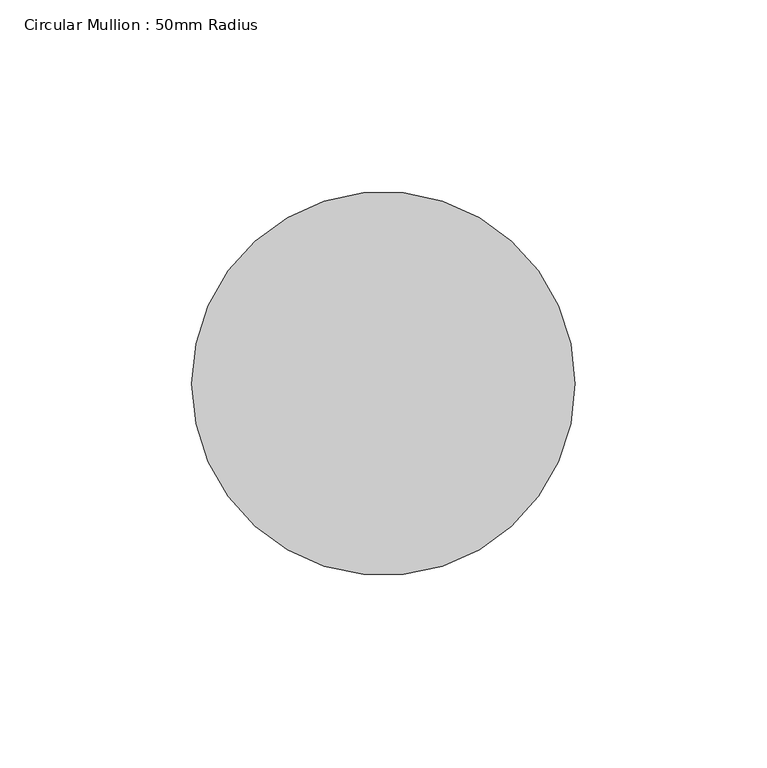
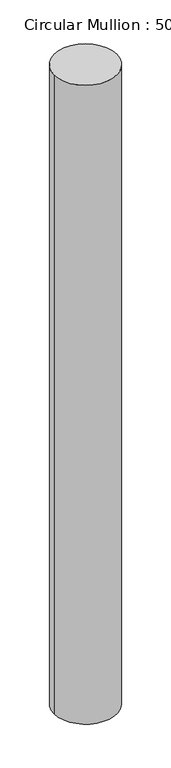
"""IFC4 building model written with IfcOpenShell, lengths in millimetres: member geometry, Circular Mullion : 50mm Radius."""

from ifc_helpers import new_model, si_unit, point, frame, origin, origin_2d, place, context, project, spatial, circle_curve, trimmed, segment, composite_curve, outline, extrude, source, transform, mapped, element, save


def circular_mullion_50mm_radius_108bae4b(model_context):
    return source(origin(), model_context, "Body", "SweptSolid", [
        extrude(outline(composite_curve([segment(trimmed(circle_curve(origin_2d(), 50.0), [point((50.0, 0.0))], [point((-50.0, 0.0))], False, "CARTESIAN"), True, "CONTINUOUS"), segment(trimmed(circle_curve(origin_2d(), 50.0), [point((-50.0, 0.0))], [point((50.0, 0.0))], False, "CARTESIAN"), True, "CONTINUOUS")], self_intersect=False)), frame((0.0, 0.0, -1076.8079908), z_axis=(0.0, 0.0, 1.0), x_axis=(1.0, 0.0, 0.0)), (0.0, 0.0, 1.0), 1076.8079908),
    ])


if __name__ == "__main__":
    model = new_model("IFC4")
    model_context = context("Model", 3, world=origin())
    ifc_project = project(units=[si_unit("LENGTHUNIT", "METRE", prefix="MILLI")], contexts=[model_context])
    site = spatial("IfcSite", under=ifc_project)
    building = spatial("IfcBuilding", under=site)
    placement = place(None, origin())
    circular_mullion_50mm_radius_shape = circular_mullion_50mm_radius_108bae4b(model_context)
    element("IfcMember", 1, ObjectType="Circular Mullion : 50mm Radius", at=placement, inside=building, context=model_context, shape_type="MappedRepresentation", body=[
        mapped(circular_mullion_50mm_radius_shape, transform((0.0, 0.0, 0.0), x_axis=(1.0, 0.0, 0.0), y_axis=(0.0, 1.0, 0.0), z_axis=(0.0, 0.0, 1.0))),
    ])
    save(model, "model.ifc")

# Revit data of these elements
# Type "Circular Mullion : 50mm Radius"
#   built-in parameter 1007350 = 0.164042 (stored number, unit not read)
# Element 1 (IfcMember, "Circular Mullion : 50mm Radius")
#   Materials on its faces: "Aluminium"
# Materials
#   "Aluminium": class "Metal", colour RGB 247 247 247, transparency 0, Description = "Aluminium 6061", Cost = 0
